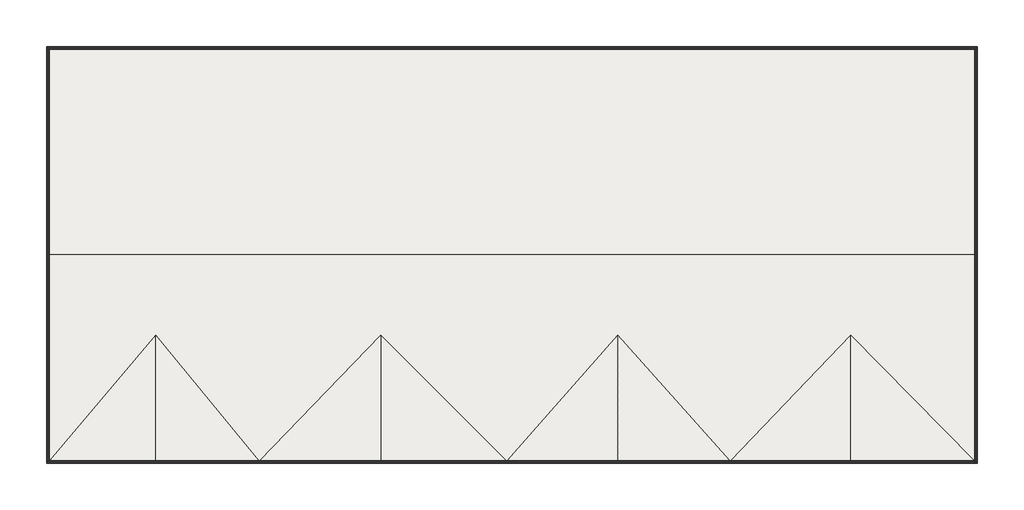
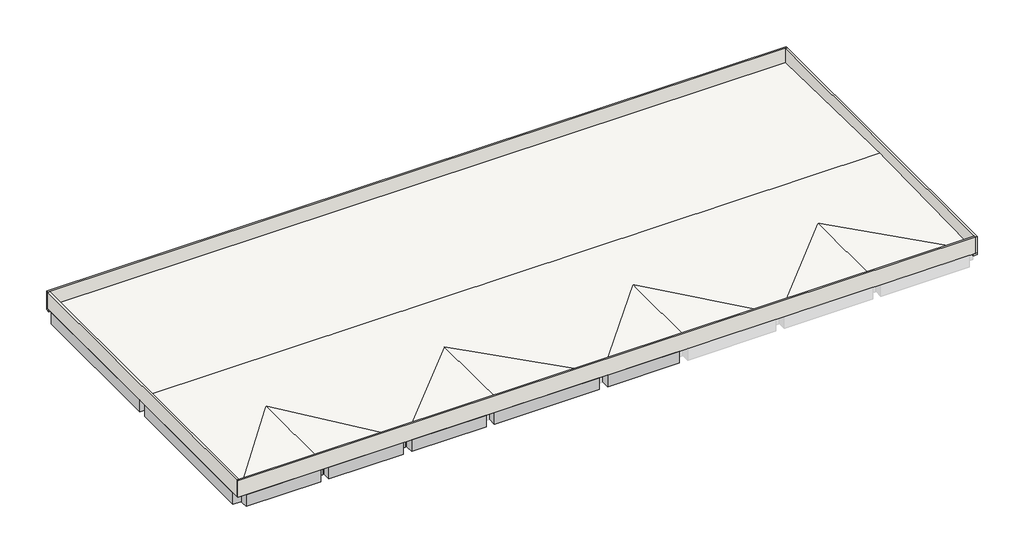
# One storey, part 1 of 2: 15 beams, 4 walls, 1 roof, 1 slab.
"""IFC4 building model written with IfcOpenShell, lengths in millimetres."""

from ifc_helpers import new_model, si_unit, frame, origin, place, context, project, spatial, polyline, outline, extrude, faceted_brep, element, save

model = new_model("IFC4")

# Units and contexts
model_context = context("Model", 3, world=origin())
ifc_project = project(units=[si_unit("LENGTHUNIT", "METRE", prefix="MILLI")], contexts=[model_context])

# Site, building, storey
site = spatial("IfcSite", under=ifc_project)
building = spatial("IfcBuilding", under=site)
storey = spatial("IfcBuildingStorey", under=building, Name="TOC", Elevation=104550.0)

# Beams
placement = place(None, origin())
element("IfcBeam", 1, ObjectType="RC Beam_Rectangular : H_SB_AR S16_RC Beam-AG_600x900_RG9", at=placement, inside=storey, context=model_context, shape_type="Brep", body=[
    faceted_brep([(300.0, -19200.0, 104550.0), (300.0, -19800.0, 104550.0), (5700.0, -19800.0, 104550.0), (5700.0, -19200.0, 104550.0), (3200.0, -19200.0, 104550.0), (2800.0, -19200.0, 104550.0), (300.0, -19800.0, 103650.0), (5700.0, -19800.0, 103650.0), (300.0, -19350.0, 103650.0), (300.0, -19200.0, 103650.0), (2800.0, -19200.0, 103650.0), (3200.0, -19200.0, 103650.0), (5700.0, -19200.0, 103650.0), (300.0, -19200.0, 104400.0)], [[[0, 1, 2, 3, 4, 5]], [[1, 6, 7, 2]], [[6, 8, 9, 10, 11, 12, 7]], [[9, 13, 0, 5, 4, 3, 12, 11, 10]], [[1, 0, 13, 9, 8, 6]], [[3, 2, 7, 12]]]),
])
element("IfcBeam", 2, ObjectType="RC Beam_Rectangular : H_SB_AR S16_RC Beam-AG_600x900_RG9", at=placement, inside=storey, context=model_context, shape_type="Brep", body=[
    faceted_brep([(6300.0, -19200.0, 104550.0), (6300.0, -19800.0, 104550.0), (11700.0, -19800.0, 104550.0), (11700.0, -19200.0, 104550.0), (9200.0, -19200.0, 104550.0), (8800.0, -19200.0, 104550.0), (6300.0, -19800.0, 103650.0), (11700.0, -19800.0, 103650.0), (6300.0, -19200.0, 103650.0), (8800.0, -19200.0, 103650.0), (9200.0, -19200.0, 103650.0), (11700.0, -19200.0, 103650.0)], [[[0, 1, 2, 3, 4, 5]], [[1, 6, 7, 2]], [[6, 8, 9, 10, 11, 7]], [[8, 0, 5, 4, 3, 11, 10, 9]], [[1, 0, 8, 6]], [[3, 2, 7, 11]]]),
])
element("IfcBeam", 3, ObjectType="RC Beam_Rectangular : H_SB_AR S16_RC Beam-AG_600x900_RG9", at=placement, inside=storey, context=model_context, shape_type="Brep", body=[
    faceted_brep([(12300.0, -19200.0, 104550.0), (12300.0, -19800.0, 104550.0), (17700.0, -19800.0, 104550.0), (17700.0, -19200.0, 104550.0), (15200.0, -19200.0, 104550.0), (14800.0, -19200.0, 104550.0), (12300.0, -19800.0, 103650.0), (17700.0, -19800.0, 103650.0), (12300.0, -19200.0, 103650.0), (14800.0, -19200.0, 103650.0), (15200.0, -19200.0, 103650.0), (17700.0, -19200.0, 103650.0), (17700.0, -19200.0, 104400.0)], [[[0, 1, 2, 3, 4, 5]], [[1, 6, 7, 2]], [[6, 8, 9, 10, 11, 7]], [[8, 0, 5, 4, 3, 12, 11, 10, 9]], [[1, 0, 8, 6]], [[3, 2, 7, 11, 12]]]),
])
element("IfcBeam", 4, ObjectType="RC Beam_Rectangular : H_SB_AR S16_RC Beam-AG_600x900_RG9", at=placement, inside=storey, context=model_context, shape_type="Brep", body=[
    faceted_brep([(18300.0, -19200.0, 104550.0), (18300.0, -19800.0, 104550.0), (25900.0, -19800.0, 104550.0), (25900.0, -19200.0, 104550.0), (22400.0, -19200.0, 104550.0), (21800.0, -19200.0, 104550.0), (25900.0, -19800.0, 103650.0), (18300.0, -19800.0, 103650.0), (18300.0, -19200.0, 103650.0), (21800.0, -19200.0, 103650.0), (22400.0, -19200.0, 103650.0), (25900.0, -19200.0, 103650.0), (18300.0, -19200.0, 104400.0)], [[[0, 1, 2, 3, 4, 5]], [[6, 2, 1, 7]], [[7, 8, 9, 10, 11, 6]], [[8, 12, 0, 5, 4, 3, 11, 10, 9]], [[0, 12, 8, 7, 1]], [[3, 2, 6, 11]]]),
])
element("IfcBeam", 5, ObjectType="RC Beam_Rectangular : H_SB_AR S16_RC Beam-AG_600x900_RG9", at=placement, inside=storey, context=model_context, shape_type="Brep", body=[
    faceted_brep([(26500.0, -19200.0, 104550.0), (26500.0, -19800.0, 104550.0), (31700.0, -19800.0, 104550.0), (31700.0, -19200.0, 104550.0), (29400.0, -19200.0, 104550.0), (28800.0, -19200.0, 104550.0), (26500.0, -19800.0, 103650.0), (31700.0, -19800.0, 103650.0), (26500.0, -19200.0, 103650.0), (28800.0, -19200.0, 103650.0), (29400.0, -19200.0, 103650.0), (31700.0, -19200.0, 103650.0)], [[[0, 1, 2, 3, 4, 5]], [[1, 6, 7, 2]], [[6, 8, 9, 10, 11, 7]], [[8, 0, 5, 4, 3, 11, 10, 9]], [[1, 0, 8, 6]], [[3, 2, 7, 11]]]),
])
element("IfcBeam", 6, ObjectType="RC Beam_Rectangular : H_SB_AR S16_RC Beam-AG_600x900_RG6", at=placement, inside=storey, context=model_context, shape_type="Brep", body=[
    faceted_brep([(-300.0, -19200.0, 104550.0), (300.0, -19200.0, 104550.0), (300.0, -8100.0, 104550.0), (-300.0, -8100.0, 104550.0), (300.0, -19200.0, 104400.0), (300.0, -19200.0, 103650.0), (300.0, -8100.0, 103650.0), (300.0, -8100.0, 104400.0), (150.0, -19200.0, 103650.0), (-300.0, -19200.0, 103650.0), (-300.0, -8100.0, 103650.0)], [[[0, 1, 2, 3]], [[1, 4, 5, 6, 7, 2]], [[5, 8, 9, 10, 6]], [[9, 0, 3, 10]], [[5, 4, 1, 0, 9, 8]], [[3, 2, 7, 6, 10]]]),
])
element("IfcBeam", 7, ObjectType="RC Beam_Rectangular : H_SB_AR S16_RC Beam-AG_600x900_RG6", at=placement, inside=storey, context=model_context, shape_type="Brep", body=[
    faceted_brep([(300.0, 3600.0, 104550.0), (-300.0, 3600.0, 104550.0), (-300.0, -7500.0, 104550.0), (300.0, -7500.0, 104550.0), (300.0, 3600.0, 103650.0), (300.0, 3600.0, 104400.0), (300.0, -7500.0, 104400.0), (300.0, -7500.0, 103650.0), (-300.0, 3600.0, 103650.0), (150.0, 3600.0, 103650.0), (-300.0, -7500.0, 103650.0)], [[[0, 1, 2, 3]], [[4, 5, 0, 3, 6, 7]], [[8, 9, 4, 7, 10]], [[10, 2, 1, 8]], [[0, 5, 4, 9, 8, 1]], [[3, 2, 10, 7, 6]]]),
])
element("IfcBeam", 8, ObjectType="RC Beam_Rectangular : H_SB_AR S16_RC Beam-AG_600x900_RG4", at=placement, inside=storey, context=model_context, shape_type="Brep", body=[
    faceted_brep([(300.0, -7500.0, 104550.0), (300.0, -8100.0, 104550.0), (2800.0, -8100.0, 104550.0), (3200.0, -8100.0, 104550.0), (5700.0, -8100.0, 104550.0), (5700.0, -7500.0, 104550.0), (3200.0, -7500.0, 104550.0), (2800.0, -7500.0, 104550.0), (300.0, -8100.0, 104400.0), (300.0, -8100.0, 103650.0), (2800.0, -8100.0, 103650.0), (3200.0, -8100.0, 103650.0), (5700.0, -8100.0, 103650.0), (300.0, -7900.0, 103650.0), (300.0, -7500.0, 103650.0), (2800.0, -7500.0, 103650.0), (3200.0, -7500.0, 103650.0), (5700.0, -7500.0, 103650.0), (300.0, -7500.0, 104400.0)], [[[0, 1, 2, 3, 4, 5, 6, 7]], [[1, 8, 9, 10, 11, 12, 4, 3, 2]], [[9, 13, 14, 15, 16, 17, 12, 11, 10]], [[14, 18, 0, 7, 6, 5, 17, 16, 15]], [[9, 8, 1, 0, 18, 14, 13]], [[5, 4, 12, 17]]]),
])
element("IfcBeam", 9, ObjectType="RC Beam_Rectangular : H_SB_AR S16_RC Beam-AG_400x900_RG1", at=placement, inside=storey, context=model_context, shape_type="Brep", body=[
    faceted_brep([(6200.0, -8100.0, 104550.0), (5800.0, -8100.0, 104550.0), (5800.0, -19200.0, 104550.0), (6200.0, -19200.0, 104550.0), (6200.0, -19200.0, 104400.0), (6200.0, -19200.0, 103650.0), (6200.0, -8100.0, 103650.0), (6200.0, -8100.0, 104400.0), (5800.0, -19200.0, 103650.0), (5800.0, -8100.0, 103650.0), (5800.0, -19200.0, 104400.0), (5800.0, -8100.0, 104400.0)], [[[0, 1, 2, 3]], [[3, 4, 5, 6, 7, 0]], [[8, 9, 6, 5]], [[8, 10, 2, 1, 11, 9]], [[2, 10, 8, 5, 4, 3]], [[0, 7, 6, 9, 11, 1]]]),
])
element("IfcBeam", 10, ObjectType="RC Beam_Rectangular : H_SB_AR S16_RC Beam-AG_400x900_RG1", at=placement, inside=storey, context=model_context, shape_type="Brep", body=[
    faceted_brep([(6200.0, 3600.0, 104550.0), (5800.0, 3600.0, 104550.0), (5800.0, -7500.0, 104550.0), (6200.0, -7500.0, 104550.0), (6200.0, -7500.0, 104400.0), (6200.0, -7500.0, 103650.0), (6200.0, 3600.0, 103650.0), (6200.0, 3600.0, 104400.0), (5800.0, -7500.0, 103650.0), (5800.0, 3600.0, 103650.0), (5800.0, -7500.0, 104400.0), (5800.0, 3600.0, 104400.0)], [[[0, 1, 2, 3]], [[3, 4, 5, 6, 7, 0]], [[8, 9, 6, 5]], [[8, 10, 2, 1, 11, 9]], [[2, 10, 8, 5, 4, 3]], [[0, 7, 6, 9, 11, 1]]]),
])
element("IfcBeam", 11, ObjectType="RC Beam_Rectangular : H_SB_AR S16_RC Beam-AG_400x900_RG1", at=placement, inside=storey, context=model_context, shape_type="Brep", body=[
    faceted_brep([(12200.0, -8100.0, 104550.0), (11800.0, -8100.0, 104550.0), (11800.0, -19200.0, 104550.0), (12200.0, -19200.0, 104550.0), (12200.0, -19200.0, 104400.0), (12200.0, -19200.0, 103650.0), (12200.0, -8100.0, 103650.0), (12200.0, -8100.0, 104400.0), (11800.0, -19200.0, 103650.0), (11800.0, -8100.0, 103650.0), (11800.0, -19200.0, 104400.0), (11800.0, -8100.0, 104400.0)], [[[0, 1, 2, 3]], [[3, 4, 5, 6, 7, 0]], [[8, 9, 6, 5]], [[8, 10, 2, 1, 11, 9]], [[2, 10, 8, 5, 4, 3]], [[0, 7, 6, 9, 11, 1]]]),
])
element("IfcBeam", 12, ObjectType="RC Beam_Rectangular : H_SB_AR S16_RC Beam-AG_400x900_RB1", at=placement, inside=storey, context=model_context, shape_type="Brep", body=[
    faceted_brep([(3200.0, 3600.0, 104550.0), (2800.0, 3600.0, 104550.0), (2800.0, -7500.0, 104550.0), (3200.0, -7500.0, 104550.0), (2800.0, 3600.0, 104400.0), (2800.0, 3600.0, 103650.0), (2800.0, -7500.0, 103650.0), (2800.0, -7500.0, 104400.0), (3200.0, 3600.0, 103650.0), (3200.0, -7500.0, 103650.0), (3200.0, 3600.0, 104400.0), (3200.0, -7500.0, 104400.0)], [[[0, 1, 2, 3]], [[1, 4, 5, 6, 7, 2]], [[5, 8, 9, 6]], [[8, 10, 0, 3, 11, 9]], [[1, 0, 10, 8, 5, 4]], [[3, 2, 7, 6, 9, 11]]]),
])
element("IfcBeam", 13, ObjectType="RC Beam_Rectangular : H_SB_AR S16_RC Beam-AG_400x900_RB1", at=placement, inside=storey, context=model_context, shape_type="Brep", body=[
    faceted_brep([(2800.0, -19200.0, 104550.0), (3200.0, -19200.0, 104550.0), (3200.0, -8100.0, 104550.0), (2800.0, -8100.0, 104550.0), (2800.0, -19200.0, 103650.0), (2800.0, -19200.0, 104400.0), (2800.0, -8100.0, 104400.0), (2800.0, -8100.0, 103650.0), (3200.0, -19200.0, 103650.0), (3200.0, -8100.0, 103650.0), (3200.0, -19200.0, 104400.0), (3200.0, -8100.0, 104400.0)], [[[0, 1, 2, 3]], [[4, 5, 0, 3, 6, 7]], [[8, 4, 7, 9]], [[1, 10, 8, 9, 11, 2]], [[1, 0, 5, 4, 8, 10]], [[3, 2, 11, 9, 7, 6]]]),
])
element("IfcBeam", 14, ObjectType="RC Beam_Rectangular : H_SB_AR S16_RC Beam-AG_400x900_RB1", at=placement, inside=storey, context=model_context, shape_type="Brep", body=[
    faceted_brep([(8800.0, -19200.0, 104550.0), (9200.0, -19200.0, 104550.0), (9200.0, -8100.0, 104550.0), (8800.0, -8100.0, 104550.0), (8800.0, -19200.0, 103650.0), (8800.0, -19200.0, 104400.0), (8800.0, -8100.0, 104400.0), (8800.0, -8100.0, 103650.0), (9200.0, -19200.0, 103650.0), (9200.0, -8100.0, 103650.0), (9200.0, -19200.0, 104400.0), (9200.0, -8100.0, 104400.0)], [[[0, 1, 2, 3]], [[4, 5, 0, 3, 6, 7]], [[8, 4, 7, 9]], [[1, 10, 8, 9, 11, 2]], [[1, 0, 5, 4, 8, 10]], [[3, 2, 11, 9, 7, 6]]]),
])
element("IfcBeam", 15, ObjectType="RC Beam_Rectangular : H_SB_AR S16_RC Beam-AG_400x900_RB1", at=placement, inside=storey, context=model_context, shape_type="Brep", body=[
    faceted_brep([(14800.0, -19200.0, 104550.0), (15200.0, -19200.0, 104550.0), (15200.0, -8100.0, 104550.0), (14800.0, -8100.0, 104550.0), (14800.0, -19200.0, 103650.0), (14800.0, -19200.0, 104400.0), (14800.0, -8100.0, 104400.0), (14800.0, -8100.0, 103650.0), (15200.0, -19200.0, 103650.0), (15200.0, -8100.0, 103650.0), (15200.0, -19200.0, 104400.0), (15200.0, -8100.0, 104400.0)], [[[0, 1, 2, 3]], [[4, 5, 0, 3, 6, 7]], [[8, 4, 7, 9]], [[1, 10, 8, 9, 11, 2]], [[1, 0, 5, 4, 8, 10]], [[3, 2, 11, 9, 7, 6]]]),
])

# Roof
element("IfcRoof", 16, ObjectType="H_RF_AR B06_RC Roof Finish_Type1", at=placement, inside=storey, context=model_context, shape_type="Brep", body=[
    faceted_brep([(53150.0, -19650.0, 104550.0), (-150.0, -19650.0, 104550.0), (-150.0, 4050.0, 104550.0), (53150.0, 4050.0, 104550.0), (-150.0, -19650.0, 104720.0), (53150.0, -19650.0, 104720.0), (46000.0, -19650.0, 104866.0), (39071.6723549, -19650.0, 104720.0), (32600.0, -19650.0, 104866.0), (26200.0, -19650.0, 104720.0), (18950.0, -19650.0, 104866.0), (11938.5665529, -19650.0, 104720.0), (6000.0, -19650.0, 104866.0), (-150.0, 4050.0, 104720.0), (-150.0, -7800.0, 104959.0), (53150.0, 4050.0, 104720.0), (53150.0, -7800.0, 104959.0), (6000.0, -12400.0, 104866.2236287), (18950.0, -12400.0, 104866.2236287), (32600.0, -12400.0, 104866.2236287), (46000.0, -12400.0, 104866.2236287)], [[[0, 1, 2, 3]], [[4, 1, 0, 5, 6, 7, 8, 9, 10, 11, 12]], [[13, 2, 1, 4, 14]], [[15, 3, 2, 13]], [[5, 0, 3, 15, 16]], [[5, 16, 14, 4, 17, 11, 18, 9, 19, 7, 20]], [[15, 13, 14, 16]], [[5, 20, 6]], [[20, 7, 6]], [[4, 12, 17]], [[17, 12, 11]], [[11, 10, 18]], [[18, 10, 9]], [[9, 8, 19]], [[7, 19, 8]]]),
])

# Slab
element("IfcSlab", 17, ObjectType="H_FL_AR_S17_RC Slab_RS1 T150", at=placement, inside=storey, context=model_context, shape_type="Brep", body=[
    faceted_brep([(-300.0, 4200.0, 104400.0), (0.0, 4200.0, 104400.0), (0.0, 3900.0, 104400.0), (-300.0, 3900.0, 104400.0), (0.0, 4200.0, 104550.0), (-300.0, 4200.0, 104550.0), (-300.0, 3900.0, 104550.0), (0.0, 3900.0, 104550.0)], [[[0, 1, 2, 3]], [[4, 5, 6, 7]], [[5, 0, 3, 6]], [[0, 5, 4, 1]], [[1, 4, 7, 2]], [[3, 2, 7, 6]]]),
    faceted_brep([(53300.0, -19800.0, 104400.0), (53000.0, -19800.0, 104400.0), (53000.0, -19500.0, 104400.0), (53300.0, -19500.0, 104400.0), (53000.0, -19800.0, 104550.0), (53300.0, -19800.0, 104550.0), (53300.0, -19500.0, 104550.0), (53000.0, -19500.0, 104550.0)], [[[0, 1, 2, 3]], [[4, 5, 6, 7]], [[0, 5, 4, 1]], [[5, 0, 3, 6]], [[1, 4, 7, 2]], [[3, 2, 7, 6]]]),
    faceted_brep([(53300.0, 4200.0, 104400.0), (53300.0, 3900.0, 104400.0), (53000.0, 3900.0, 104400.0), (53000.0, 4200.0, 104400.0), (53300.0, 3900.0, 104550.0), (53300.0, 4200.0, 104550.0), (53000.0, 4200.0, 104550.0), (53000.0, 3900.0, 104550.0)], [[[0, 1, 2, 3]], [[4, 5, 6, 7]], [[5, 0, 3, 6]], [[0, 5, 4, 1]], [[6, 3, 2, 7]], [[2, 1, 4, 7]]]),
    faceted_brep([(17700.0, -8100.0, 104400.0), (17700.0, -19200.0, 104400.0), (15200.0, -19200.0, 104400.0), (15200.0, -8100.0, 104400.0), (15200.0, -19200.0, 104550.0), (17700.0, -19200.0, 104550.0), (17700.0, -8100.0, 104550.0), (15200.0, -8100.0, 104550.0)], [[[0, 1, 2, 3]], [[4, 5, 6, 7]], [[1, 5, 4, 2]], [[5, 1, 0, 6]], [[6, 0, 3, 7]], [[3, 2, 4, 7]]]),
    faceted_brep([(17700.0, 3600.0, 104400.0), (17700.0, -7500.0, 104400.0), (15200.0, -7500.0, 104400.0), (15200.0, 3600.0, 104400.0), (17700.0, -7500.0, 104550.0), (17700.0, 3600.0, 104550.0), (15200.0, 3600.0, 104550.0), (15200.0, -7500.0, 104550.0)], [[[0, 1, 2, 3]], [[4, 5, 6, 7]], [[5, 0, 3, 6]], [[1, 4, 7, 2]], [[1, 0, 5, 4]], [[3, 2, 7, 6]]]),
    faceted_brep([(6200.0, -19200.0, 104400.0), (6200.0, -8100.0, 104400.0), (8800.0, -8100.0, 104400.0), (8800.0, -19200.0, 104400.0), (6200.0, -8100.0, 104550.0), (6200.0, -19200.0, 104550.0), (6300.0, -19200.0, 104550.0), (8800.0, -19200.0, 104550.0), (8800.0, -8100.0, 104550.0), (6300.0, -8100.0, 104550.0)], [[[0, 1, 2, 3]], [[4, 5, 6, 7, 8, 9]], [[5, 0, 3, 7, 6]], [[1, 4, 9, 8, 2]], [[1, 0, 5, 4]], [[3, 2, 8, 7]]]),
    faceted_brep([(5800.0, -8100.0, 104400.0), (5800.0, -19200.0, 104400.0), (3200.0, -19200.0, 104400.0), (3200.0, -8100.0, 104400.0), (5800.0, -19200.0, 104550.0), (5800.0, -8100.0, 104550.0), (5700.0, -8100.0, 104550.0), (3200.0, -8100.0, 104550.0), (3200.0, -19200.0, 104550.0), (5700.0, -19200.0, 104550.0)], [[[0, 1, 2, 3]], [[4, 5, 6, 7, 8, 9]], [[1, 4, 9, 8, 2]], [[5, 0, 3, 7, 6]], [[1, 0, 5, 4]], [[3, 2, 8, 7]]]),
    faceted_brep([(6200.0, -7500.0, 104400.0), (6200.0, 3600.0, 104400.0), (8800.0, 3600.0, 104400.0), (8800.0, -7500.0, 104400.0), (6200.0, 3600.0, 104550.0), (6200.0, -7500.0, 104550.0), (6300.0, -7500.0, 104550.0), (8800.0, -7500.0, 104550.0), (8800.0, 3600.0, 104550.0), (6300.0, 3600.0, 104550.0)], [[[0, 1, 2, 3]], [[4, 5, 6, 7, 8, 9]], [[1, 4, 9, 8, 2]], [[5, 0, 3, 7, 6]], [[1, 0, 5, 4]], [[3, 2, 8, 7]]]),
    faceted_brep([(5800.0, 3600.0, 104400.0), (5800.0, -7500.0, 104400.0), (3200.0, -7500.0, 104400.0), (3200.0, 3600.0, 104400.0), (5800.0, -7500.0, 104550.0), (5800.0, 3600.0, 104550.0), (5700.0, 3600.0, 104550.0), (3200.0, 3600.0, 104550.0), (3200.0, -7500.0, 104550.0), (5700.0, -7500.0, 104550.0)], [[[0, 1, 2, 3]], [[4, 5, 6, 7, 8, 9]], [[5, 0, 3, 7, 6]], [[1, 4, 9, 8, 2]], [[1, 0, 5, 4]], [[3, 2, 8, 7]]]),
    faceted_brep([(12200.0, -19200.0, 104400.0), (12200.0, -8100.0, 104400.0), (14800.0, -8100.0, 104400.0), (14800.0, -19200.0, 104400.0), (12200.0, -8100.0, 104550.0), (12200.0, -19200.0, 104550.0), (12300.0, -19200.0, 104550.0), (14800.0, -19200.0, 104550.0), (14800.0, -8100.0, 104550.0), (12300.0, -8100.0, 104550.0)], [[[0, 1, 2, 3]], [[4, 5, 6, 7, 8, 9]], [[5, 0, 3, 7, 6]], [[1, 4, 9, 8, 2]], [[1, 0, 5, 4]], [[3, 2, 8, 7]]]),
    faceted_brep([(11800.0, -8100.0, 104400.0), (11800.0, -19200.0, 104400.0), (9200.0, -19200.0, 104400.0), (9200.0, -8100.0, 104400.0), (11800.0, -19200.0, 104550.0), (11800.0, -8100.0, 104550.0), (11700.0, -8100.0, 104550.0), (9200.0, -8100.0, 104550.0), (9200.0, -19200.0, 104550.0), (11700.0, -19200.0, 104550.0)], [[[0, 1, 2, 3]], [[4, 5, 6, 7, 8, 9]], [[1, 4, 9, 8, 2]], [[5, 0, 3, 7, 6]], [[1, 0, 5, 4]], [[3, 2, 8, 7]]]),
    faceted_brep([(12200.0, -7500.0, 104400.0), (12200.0, 3600.0, 104400.0), (14800.0, 3600.0, 104400.0), (14800.0, -7500.0, 104400.0), (12200.0, 3600.0, 104550.0), (12200.0, -7500.0, 104550.0), (12300.0, -7500.0, 104550.0), (14800.0, -7500.0, 104550.0), (14800.0, 3600.0, 104550.0), (12300.0, 3600.0, 104550.0)], [[[0, 1, 2, 3]], [[4, 5, 6, 7, 8, 9]], [[1, 4, 9, 8, 2]], [[5, 0, 3, 7, 6]], [[1, 0, 5, 4]], [[3, 2, 8, 7]]]),
    faceted_brep([(11800.0, 3600.0, 104400.0), (11800.0, -7500.0, 104400.0), (9200.0, -7500.0, 104400.0), (9200.0, 3600.0, 104400.0), (11800.0, -7500.0, 104550.0), (11800.0, 3600.0, 104550.0), (11700.0, 3600.0, 104550.0), (9200.0, 3600.0, 104550.0), (9200.0, -7500.0, 104550.0), (11700.0, -7500.0, 104550.0)], [[[0, 1, 2, 3]], [[4, 5, 6, 7, 8, 9]], [[5, 0, 3, 7, 6]], [[1, 4, 9, 8, 2]], [[1, 0, 5, 4]], [[3, 2, 8, 7]]]),
    faceted_brep([(2800.0, -8100.0, 104400.0), (2800.0, -19200.0, 104400.0), (426.0, -19200.0, 104400.0), (300.0, -19200.0, 104400.0), (300.0, -8100.0, 104400.0), (426.0, -8100.0, 104400.0), (300.0, -19200.0, 104550.0), (2800.0, -19200.0, 104550.0), (2800.0, -8100.0, 104550.0), (300.0, -8100.0, 104550.0)], [[[0, 1, 2, 3, 4, 5]], [[6, 7, 8, 9]], [[6, 3, 2, 1, 7]], [[3, 6, 9, 4]], [[4, 9, 8, 0, 5]], [[1, 0, 8, 7]]]),
    faceted_brep([(25950.0, 3600.0, 104400.0), (25950.0, -11400.0, 104400.0), (22400.0, -11400.0, 104400.0), (22400.0, 3600.0, 104400.0), (25950.0, -11400.0, 104550.0), (25950.0, 3600.0, 104550.0), (25900.0, 3600.0, 104550.0), (22400.0, 3600.0, 104550.0), (22400.0, -11400.0, 104550.0), (25900.0, -11400.0, 104550.0)], [[[0, 1, 2, 3]], [[4, 5, 6, 7, 8, 9]], [[5, 0, 3, 7, 6]], [[1, 4, 9, 8, 2]], [[1, 0, 5, 4]], [[3, 2, 8, 7]]]),
    faceted_brep([(26450.0, -11400.0, 104400.0), (26450.0, 3600.0, 104400.0), (28800.0, 3600.0, 104400.0), (28800.0, -11400.0, 104400.0), (26450.0, 3600.0, 104550.0), (26450.0, -11400.0, 104550.0), (26500.0, -11400.0, 104550.0), (28800.0, -11400.0, 104550.0), (28800.0, 3600.0, 104550.0), (26500.0, 3600.0, 104550.0)], [[[0, 1, 2, 3]], [[4, 5, 6, 7, 8, 9]], [[1, 4, 9, 8, 2]], [[5, 0, 3, 7, 6]], [[1, 0, 5, 4]], [[3, 2, 8, 7]]]),
    faceted_brep([(25950.0, -12000.0, 104400.0), (25950.0, -19200.0, 104400.0), (22400.0, -19200.0, 104400.0), (22400.0, -12000.0, 104400.0), (25950.0, -19200.0, 104550.0), (25950.0, -12000.0, 104550.0), (25900.0, -12000.0, 104550.0), (22400.0, -12000.0, 104550.0), (22400.0, -19200.0, 104550.0), (25900.0, -19200.0, 104550.0)], [[[0, 1, 2, 3]], [[4, 5, 6, 7, 8, 9]], [[1, 4, 9, 8, 2]], [[5, 0, 3, 7, 6]], [[1, 0, 5, 4]], [[3, 2, 8, 7]]]),
    faceted_brep([(31750.0, 3600.0, 104400.0), (31750.0, -11400.0, 104400.0), (29400.0, -11400.0, 104400.0), (29400.0, 3600.0, 104400.0), (31750.0, -11400.0, 104550.0), (31750.0, 3600.0, 104550.0), (31700.0, 3600.0, 104550.0), (29400.0, 3600.0, 104550.0), (29400.0, -11400.0, 104550.0), (31700.0, -11400.0, 104550.0)], [[[0, 1, 2, 3]], [[4, 5, 6, 7, 8, 9]], [[5, 0, 3, 7, 6]], [[1, 4, 9, 8, 2]], [[1, 0, 5, 4]], [[3, 2, 8, 7]]]),
    faceted_brep([(32250.0, -11400.0, 104400.0), (32250.0, 3600.0, 104400.0), (33250.0, 3600.0, 104400.0), (33450.0, 3600.0, 104400.0), (35200.0, 3600.0, 104400.0), (35200.0, -11400.0, 104400.0), (33450.0, -11400.0, 104400.0), (33250.0, -11400.0, 104400.0), (32250.0, 3600.0, 104550.0), (32250.0, -11400.0, 104550.0), (32300.0, -11400.0, 104550.0), (35200.0, -11400.0, 104550.0), (35200.0, 3600.0, 104550.0), (32300.0, 3600.0, 104550.0)], [[[0, 1, 2, 3, 4, 5, 6, 7]], [[8, 9, 10, 11, 12, 13]], [[1, 8, 13, 12, 4, 3, 2]], [[9, 0, 7, 6, 5, 11, 10]], [[1, 0, 9, 8]], [[5, 4, 12, 11]]]),
    faceted_brep([(32250.0, -19200.0, 104400.0), (32250.0, -12000.0, 104400.0), (35200.0, -12000.0, 104400.0), (35200.0, -19200.0, 104400.0), (32250.0, -12000.0, 104550.0), (32250.0, -19200.0, 104550.0), (32300.0, -19200.0, 104550.0), (35200.0, -19200.0, 104550.0), (35200.0, -12000.0, 104550.0), (32300.0, -12000.0, 104550.0)], [[[0, 1, 2, 3]], [[4, 5, 6, 7, 8, 9]], [[5, 0, 3, 7, 6]], [[1, 4, 9, 8, 2]], [[1, 0, 5, 4]], [[3, 2, 8, 7]]]),
    faceted_brep([(26450.0, -19200.0, 104400.0), (26450.0, -12000.0, 104400.0), (26500.0, -12000.0, 104400.0), (28500.0, -12000.0, 104400.0), (28700.0, -12000.0, 104400.0), (28800.0, -12000.0, 104400.0), (28800.0, -15000.0, 104400.0), (28800.0, -15200.0, 104400.0), (28800.0, -19200.0, 104400.0), (28700.0, -19200.0, 104400.0), (28500.0, -19200.0, 104400.0), (26500.0, -19200.0, 104400.0), (26450.0, -12000.0, 104550.0), (26450.0, -19200.0, 104550.0), (26500.0, -19200.0, 104550.0), (28800.0, -19200.0, 104550.0), (28800.0, -12000.0, 104550.0), (26500.0, -12000.0, 104550.0)], [[[0, 1, 2, 3, 4, 5, 6, 7, 8, 9, 10, 11]], [[12, 13, 14, 15, 16, 17]], [[13, 0, 11, 10, 9, 8, 15, 14]], [[1, 12, 17, 16, 5, 4, 3, 2]], [[1, 0, 13, 12]], [[8, 7, 6, 5, 16, 15]]]),
    faceted_brep([(31750.0, -12000.0, 104400.0), (31750.0, -19200.0, 104400.0), (31700.0, -19200.0, 104400.0), (29400.0, -19200.0, 104400.0), (29400.0, -15200.0, 104400.0), (29400.0, -15000.0, 104400.0), (29400.0, -12000.0, 104400.0), (31700.0, -12000.0, 104400.0), (31750.0, -19200.0, 104550.0), (31750.0, -12000.0, 104550.0), (31700.0, -12000.0, 104550.0), (29400.0, -12000.0, 104550.0), (29400.0, -19200.0, 104550.0), (31700.0, -19200.0, 104550.0)], [[[0, 1, 2, 3, 4, 5, 6, 7]], [[8, 9, 10, 11, 12, 13]], [[1, 8, 13, 12, 3, 2]], [[9, 0, 7, 6, 11, 10]], [[1, 0, 9, 8]], [[6, 5, 4, 3, 12, 11]]]),
    faceted_brep([(38750.0, 3600.0, 104400.0), (38750.0, -9150.0, 104400.0), (38750.0, -9350.0, 104400.0), (38750.0, -11400.0, 104400.0), (36700.0, -11400.0, 104400.0), (36500.0, -11400.0, 104400.0), (35800.0, -11400.0, 104400.0), (35800.0, 3600.0, 104400.0), (38750.0, -11400.0, 104550.0), (38750.0, 3600.0, 104550.0), (38700.0, 3600.0, 104550.0), (35800.0, 3600.0, 104550.0), (35800.0, -11400.0, 104550.0), (38700.0, -11400.0, 104550.0)], [[[0, 1, 2, 3, 4, 5, 6, 7]], [[8, 9, 10, 11, 12, 13]], [[9, 0, 7, 11, 10]], [[3, 8, 13, 12, 6, 5, 4]], [[3, 2, 1, 0, 9, 8]], [[7, 6, 12, 11]]]),
    faceted_brep([(39250.0, -11400.0, 104400.0), (39250.0, -9350.0, 104400.0), (39250.0, -9150.0, 104400.0), (39250.0, 3600.0, 104400.0), (42200.0, 3600.0, 104400.0), (42200.0, -9150.0, 104400.0), (42200.0, -9350.0, 104400.0), (42200.0, -11400.0, 104400.0), (39250.0, 3600.0, 104550.0), (39250.0, -11400.0, 104550.0), (39300.0, -11400.0, 104550.0), (42200.0, -11400.0, 104550.0), (42200.0, 3600.0, 104550.0), (39300.0, 3600.0, 104550.0)], [[[0, 1, 2, 3, 4, 5, 6, 7]], [[8, 9, 10, 11, 12, 13]], [[3, 8, 13, 12, 4]], [[9, 0, 7, 11, 10]], [[3, 2, 1, 0, 9, 8]], [[7, 6, 5, 4, 12, 11]]]),
    faceted_brep([(38750.0, -12000.0, 104400.0), (38750.0, -19200.0, 104400.0), (38700.0, -19200.0, 104400.0), (36700.0, -19200.0, 104400.0), (36500.0, -19200.0, 104400.0), (35800.0, -19200.0, 104400.0), (35800.0, -12000.0, 104400.0), (36500.0, -12000.0, 104400.0), (36700.0, -12000.0, 104400.0), (38700.0, -12000.0, 104400.0), (38750.0, -19200.0, 104550.0), (38750.0, -12000.0, 104550.0), (38700.0, -12000.0, 104550.0), (35800.0, -12000.0, 104550.0), (35800.0, -19200.0, 104550.0), (38700.0, -19200.0, 104550.0)], [[[0, 1, 2, 3, 4, 5, 6, 7, 8, 9]], [[10, 11, 12, 13, 14, 15]], [[1, 10, 15, 14, 5, 4, 3, 2]], [[11, 0, 9, 8, 7, 6, 13, 12]], [[1, 0, 11, 10]], [[6, 5, 14, 13]]]),
    faceted_brep([(39250.0, -19200.0, 104400.0), (39250.0, -15350.0, 104400.0), (39250.0, -15150.0, 104400.0), (39250.0, -12000.0, 104400.0), (42100.0, -12000.0, 104400.0), (42200.0, -12000.0, 104400.0), (42200.0, -15150.0, 104400.0), (42200.0, -15350.0, 104400.0), (42200.0, -19200.0, 104400.0), (39250.0, -12000.0, 104550.0), (39250.0, -19200.0, 104550.0), (39300.0, -19200.0, 104550.0), (42200.0, -19200.0, 104550.0), (42200.0, -12000.0, 104550.0), (39300.0, -12000.0, 104550.0)], [[[0, 1, 2, 3, 4, 5, 6, 7, 8]], [[9, 10, 11, 12, 13, 14]], [[10, 0, 8, 12, 11]], [[3, 9, 14, 13, 5, 4]], [[3, 2, 1, 0, 10, 9]], [[8, 7, 6, 5, 13, 12]]]),
    faceted_brep([(45750.0, 3600.0, 104400.0), (45750.0, 900.0, 104400.0), (45750.0, 700.0, 104400.0), (45750.0, -9150.0, 104400.0), (45750.0, -9350.0, 104400.0), (45750.0, -11400.0, 104400.0), (42800.0, -11400.0, 104400.0), (42800.0, -9350.0, 104400.0), (42800.0, -9150.0, 104400.0), (42800.0, 3600.0, 104400.0), (43550.0, 3600.0, 104400.0), (43600.0, 3600.0, 104400.0), (43800.0, 3600.0, 104400.0), (45750.0, -11400.0, 104550.0), (45750.0, 3600.0, 104550.0), (45700.0, 3600.0, 104550.0), (42800.0, 3600.0, 104550.0), (42800.0, -11400.0, 104550.0), (45700.0, -11400.0, 104550.0)], [[[0, 1, 2, 3, 4, 5, 6, 7, 8, 9, 10, 11, 12]], [[13, 14, 15, 16, 17, 18]], [[14, 0, 12, 11, 10, 9, 16, 15]], [[5, 13, 18, 17, 6]], [[5, 4, 3, 2, 1, 0, 14, 13]], [[9, 8, 7, 6, 17, 16]]]),
    faceted_brep([(46250.0, -11400.0, 104400.0), (46250.0, -10150.0, 104400.0), (46250.0, -9950.0, 104400.0), (46250.0, -6215.0, 104400.0), (46250.0, -6015.0, 104400.0), (46250.0, -4945.0, 104400.0), (46250.0, -4745.0, 104400.0), (46250.0, -3565.0, 104400.0), (46250.0, -3365.0, 104400.0), (46250.0, -1950.0, 104400.0), (46250.0, -1750.0, 104400.0), (46250.0, -550.0, 104400.0), (46250.0, -350.0, 104400.0), (46250.0, 3600.0, 104400.0), (46600.0, 3600.0, 104400.0), (46600.0, -1750.0, 104400.0), (46600.0, -1950.0, 104400.0), (46600.0, -6015.0, 104400.0), (46600.0, -6215.0, 104400.0), (46600.0, -9950.0, 104400.0), (46600.0, -10150.0, 104400.0), (46600.0, -11400.0, 104400.0), (46250.0, 3600.0, 104550.0), (46250.0, -11400.0, 104550.0), (46300.0, -11400.0, 104550.0), (46600.0, -11400.0, 104550.0), (46600.0, 3600.0, 104550.0), (46300.0, 3600.0, 104550.0)], [[[0, 1, 2, 3, 4, 5, 6, 7, 8, 9, 10, 11, 12, 13, 14, 15, 16, 17, 18, 19, 20, 21]], [[22, 23, 24, 25, 26, 27]], [[13, 22, 27, 26, 14]], [[23, 0, 21, 25, 24]], [[13, 12, 11, 10, 9, 8, 7, 6, 5, 4, 3, 2, 1, 0, 23, 22]], [[21, 20, 19, 18, 17, 16, 15, 14, 26, 25]]]),
    faceted_brep([(45750.0, -12000.0, 104400.0), (45750.0, -13200.0, 104400.0), (45750.0, -13400.0, 104400.0), (45750.0, -15150.0, 104400.0), (45750.0, -15350.0, 104400.0), (45750.0, -19200.0, 104400.0), (43500.0, -19200.0, 104400.0), (43300.0, -19200.0, 104400.0), (43100.0, -19200.0, 104400.0), (42800.0, -19200.0, 104400.0), (42800.0, -15350.0, 104400.0), (42800.0, -15150.0, 104400.0), (42800.0, -13899.2374861, 104400.0), (42800.0, -13699.2374861, 104400.0), (42800.0, -12000.0, 104400.0), (43300.0, -12000.0, 104400.0), (43500.0, -12000.0, 104400.0), (45000.0, -12000.0, 104400.0), (45200.0, -12000.0, 104400.0), (45750.0, -19200.0, 104550.0), (45750.0, -12000.0, 104550.0), (45700.0, -12000.0, 104550.0), (42800.0, -12000.0, 104550.0), (42800.0, -19200.0, 104550.0), (45700.0, -19200.0, 104550.0)], [[[0, 1, 2, 3, 4, 5, 6, 7, 8, 9, 10, 11, 12, 13, 14, 15, 16, 17, 18]], [[19, 20, 21, 22, 23, 24]], [[5, 19, 24, 23, 9, 8, 7, 6]], [[20, 0, 18, 17, 16, 15, 14, 22, 21]], [[5, 4, 3, 2, 1, 0, 20, 19]], [[14, 13, 12, 11, 10, 9, 23, 22]]]),
    faceted_brep([(46250.0, -19200.0, 104400.0), (46250.0, -15350.0, 104400.0), (46250.0, -15150.0, 104400.0), (46250.0, -13400.0, 104400.0), (46250.0, -13200.0, 104400.0), (46250.0, -12000.0, 104400.0), (46600.0, -12000.0, 104400.0), (47200.0, -12000.0, 104400.0), (49200.0, -12000.0, 104400.0), (49200.0, -19200.0, 104400.0), (46800.0, -19200.0, 104400.0), (46600.0, -19200.0, 104400.0), (46250.0, -12000.0, 104550.0), (46250.0, -19200.0, 104550.0), (46300.0, -19200.0, 104550.0), (49200.0, -19200.0, 104550.0), (49200.0, -12000.0, 104550.0), (47200.0, -12000.0, 104550.0), (46600.0, -12000.0, 104550.0), (46300.0, -12000.0, 104550.0)], [[[0, 1, 2, 3, 4, 5, 6, 7, 8, 9, 10, 11]], [[12, 13, 14, 15, 16, 17, 18, 19]], [[13, 0, 11, 10, 9, 15, 14]], [[5, 12, 19, 18, 17, 16, 8, 7, 6]], [[5, 4, 3, 2, 1, 0, 13, 12]], [[9, 8, 16, 15]]]),
    faceted_brep([(300.0, 3600.0, 104400.0), (426.0, 3600.0, 104400.0), (2800.0, 3600.0, 104400.0), (2800.0, -7500.0, 104400.0), (300.0, -7500.0, 104400.0), (2800.0, -7500.0, 104550.0), (2800.0, 3600.0, 104550.0), (300.0, 3600.0, 104550.0), (300.0, -7500.0, 104550.0)], [[[0, 1, 2, 3, 4]], [[5, 6, 7, 8]], [[0, 7, 6, 2, 1]], [[7, 0, 4, 8]], [[8, 4, 3, 5]], [[3, 2, 6, 5]]]),
    faceted_brep([(18300.0, -11400.0, 104400.0), (18300.0, 3474.0, 104400.0), (18300.0, 3600.0, 104400.0), (21800.0, 3600.0, 104400.0), (21800.0, -11400.0, 104400.0), (21800.0, -11400.0, 104550.0), (21800.0, 3600.0, 104550.0), (18300.0, 3600.0, 104550.0), (18300.0, -7500.0, 104550.0), (18300.0, -8100.0, 104550.0), (18300.0, -11400.0, 104550.0)], [[[0, 1, 2, 3, 4]], [[5, 6, 7, 8, 9, 10]], [[2, 7, 6, 3]], [[10, 0, 4, 5]], [[0, 10, 9, 8, 7, 2, 1]], [[4, 3, 6, 5]]]),
    faceted_brep([(52700.0, 3600.0, 104400.0), (52700.0, 3474.0, 104400.0), (52700.0, -1750.0, 104400.0), (52700.0, -1950.0, 104400.0), (52700.0, -6015.0, 104400.0), (52700.0, -6215.0, 104400.0), (52700.0, -8200.0, 104400.0), (52700.0, -8400.0, 104400.0), (52700.0, -11400.0, 104400.0), (52574.0, -11400.0, 104400.0), (52374.0, -11400.0, 104400.0), (50570.0, -11400.0, 104400.0), (50370.0, -11400.0, 104400.0), (49800.0, -11400.0, 104400.0), (49200.0, -11400.0, 104400.0), (47200.0, -11400.0, 104400.0), (47200.0, -10150.0, 104400.0), (47200.0, -9950.0, 104400.0), (47200.0, -6215.0, 104400.0), (47200.0, -6015.0, 104400.0), (47200.0, -1950.0, 104400.0), (47200.0, -1750.0, 104400.0), (47200.0, 3600.0, 104400.0), (48900.0, 3600.0, 104400.0), (49100.0, 3600.0, 104400.0), (47200.0, 3600.0, 104550.0), (47200.0, -11400.0, 104550.0), (49200.0, -11400.0, 104550.0), (49800.0, -11400.0, 104550.0), (52700.0, -11400.0, 104550.0), (52700.0, 3600.0, 104550.0)], [[[0, 1, 2, 3, 4, 5, 6, 7, 8, 9, 10, 11, 12, 13, 14, 15, 16, 17, 18, 19, 20, 21, 22, 23, 24]], [[25, 26, 27, 28, 29, 30]], [[30, 0, 24, 23, 22, 25]], [[0, 30, 29, 8, 7, 6, 5, 4, 3, 2, 1]], [[8, 29, 28, 27, 26, 15, 14, 13, 12, 11, 10, 9]], [[22, 21, 20, 19, 18, 17, 16, 15, 26, 25]]]),
    faceted_brep([(52700.0, -12000.0, 104400.0), (52700.0, -19200.0, 104400.0), (52574.0, -19200.0, 104400.0), (49800.0, -19200.0, 104400.0), (49800.0, -12000.0, 104400.0), (49800.0, -19200.0, 104550.0), (52700.0, -19200.0, 104550.0), (52700.0, -12000.0, 104550.0), (49800.0, -12000.0, 104550.0)], [[[0, 1, 2, 3, 4]], [[5, 6, 7, 8]], [[1, 6, 5, 3, 2]], [[6, 1, 0, 7]], [[7, 0, 4, 8]], [[4, 3, 5, 8]]]),
    faceted_brep([(18300.0, -19200.0, 104400.0), (18300.0, -19074.0, 104400.0), (18300.0, -12000.0, 104400.0), (21800.0, -12000.0, 104400.0), (21800.0, -19200.0, 104400.0), (18300.0, -12000.0, 104550.0), (18300.0, -19200.0, 104550.0), (21800.0, -19200.0, 104550.0), (21800.0, -12000.0, 104550.0)], [[[0, 1, 2, 3, 4]], [[5, 6, 7, 8]], [[6, 0, 4, 7]], [[2, 5, 8, 3]], [[2, 1, 0, 6, 5]], [[4, 3, 8, 7]]]),
])

# Walls
element("IfcWall", 18, ObjectType="H_WA_AR B02_Ext Wall RC-AG_EW5", at=placement, inside=storey, context=model_context, shape_type="Brep", body=[
    faceted_brep([(-300.0, 4050.0, 104550.0), (-150.0, 4050.0, 104550.0), (53150.0, 4050.0, 104550.0), (53300.0, 4050.0, 104550.0), (53300.0, 4050.0, 105799.9618634), (53150.0, 4050.0, 105799.9618634), (-150.0, 4050.0, 105799.9618634), (-300.0, 4050.0, 105799.9618634), (-300.0, 4200.0, 104550.0), (-300.0, 4200.0, 105799.9618634), (53300.0, 4200.0, 105799.9618634), (53300.0, 4200.0, 104550.0)], [[[0, 1, 2, 3, 4, 5, 6, 7]], [[8, 9, 10, 11]], [[3, 2, 1, 0, 8, 11]], [[7, 6, 5, 4, 10, 9]], [[4, 3, 11, 10]], [[0, 7, 9, 8]]]),
])
element("IfcWall", 19, ObjectType="H_WA_AR B02_Ext Wall RC-AG_EW5", at=placement, inside=storey, context=model_context, shape_type="Brep", body=[
    faceted_brep([(53150.0, 4050.0, 104550.0), (53150.0, -19650.0, 104550.0), (53150.0, -19800.0, 104550.0), (53150.0, -19800.0, 105799.9618634), (53150.0, -19650.0, 105799.9618634), (53150.0, 4050.0, 105799.9618634), (53300.0, 4050.0, 104550.0), (53300.0, 4050.0, 105799.9618634), (53300.0, -19800.0, 105799.9618634), (53300.0, -19800.0, 104550.0)], [[[0, 1, 2, 3, 4, 5]], [[6, 7, 8, 9]], [[2, 1, 0, 6, 9]], [[5, 4, 3, 8, 7]], [[0, 5, 7, 6]], [[3, 2, 9, 8]]]),
])
element("IfcWall", 20, ObjectType="H_WA_AR B02_Ext Wall RC-AG_EW5", at=placement, inside=storey, context=model_context, shape_type="Brep", body=[
    faceted_brep([(53150.0, -19650.0, 104550.0), (-150.0, -19650.0, 104550.0), (-300.0, -19650.0, 104550.0), (-300.0, -19650.0, 105799.9618634), (-150.0, -19650.0, 105799.9618634), (53150.0, -19650.0, 105799.9618634), (53150.0, -19800.0, 104550.0), (53150.0, -19800.0, 105799.9618634), (-300.0, -19800.0, 105799.9618634), (-300.0, -19800.0, 104550.0)], [[[0, 1, 2, 3, 4, 5]], [[6, 7, 8, 9]], [[2, 1, 0, 6, 9]], [[5, 4, 3, 8, 7]], [[0, 5, 7, 6]], [[3, 2, 9, 8]]]),
])
element("IfcWall", 21, ObjectType="H_WA_AR B02_Ext Wall RC-AG_EW5", at=placement, inside=storey, context=model_context, shape_type="SweptSolid", body=[
    extrude(outline(polyline([(-150.0, 4050.0), (-150.0, -19650.0), (-300.0, -19650.0), (-300.0, 4050.0), (-150.0, 4050.0)])), frame((0.0, 0.0, 104550.0), z_axis=(0.0, 0.0, 1.0), x_axis=(1.0, 0.0, 0.0)), (0.0, 0.0, 1.0), 1249.9618634),
])

save(model, "model.ifc")

# Revit data of these elements
# Type "RC Beam_Rectangular : H_SB_AR S16_RC Beam-AG_600x900_RG9"
#   Type Comments = "AG"
#   Type Mark = "RG9"
#   중앙부 하부근 = ""
#   중앙부 상부근 = ""
#   중앙부 보조근 = ""
#   중앙부 늑근 = ""
#   외단부 하부근 = ""
#   외단부 상부근 = ""
#   외단부 보조근 = ""
#   외단부 늑근 = ""
#   부호 = ""
#   내단부 하부근 = ""
#   내단부 상부근 = ""
#   내단부 보조근 = ""
#   내단부 늑근 = ""
#   ALL 하부근 = ""
#   ALL 상부근 = ""
#   ALL 보조근 = ""
#   ALL 늑근 = ""
#   H_Rebar Ratio = 0.14
#   Width = 600 mm
#   Height = 900 mm
#   Length [instance default] = 1524 mm
#   b = 600 mm
#   h = 900 mm
#   hec_material3 [instance default] = none
#   hec_material2 [instance default] = none
#   hec_material1 [instance default] = none
#   Structural Material [instance default] = none
#   Assembly Code = ""
# Type "RC Beam_Rectangular : H_SB_AR S16_RC Beam-AG_600x900_RG6"
#   Type Comments = "AG"
#   Type Mark = "RG6"
#   중앙부 하부근 = ""
#   중앙부 상부근 = ""
#   중앙부 보조근 = ""
#   중앙부 늑근 = ""
#   외단부 하부근 = ""
#   외단부 상부근 = ""
#   외단부 보조근 = ""
#   외단부 늑근 = ""
#   부호 = ""
#   내단부 하부근 = ""
#   내단부 상부근 = ""
#   내단부 보조근 = ""
#   내단부 늑근 = ""
#   ALL 하부근 = ""
#   ALL 상부근 = ""
#   ALL 보조근 = ""
#   ALL 늑근 = ""
#   H_Rebar Ratio = 0.14
#   Width = 600 mm
#   Height = 900 mm
#   Length [instance default] = 1524 mm
#   b = 600 mm
#   h = 900 mm
#   hec_material3 [instance default] = none
#   hec_material2 [instance default] = none
#   hec_material1 [instance default] = none
#   Structural Material [instance default] = none
#   Assembly Code = ""
# Type "RC Beam_Rectangular : H_SB_AR S16_RC Beam-AG_600x900_RG4"
#   Type Comments = "AG"
#   Type Mark = "RG4"
#   중앙부 하부근 = ""
#   중앙부 상부근 = ""
#   중앙부 보조근 = ""
#   중앙부 늑근 = ""
#   외단부 하부근 = ""
#   외단부 상부근 = ""
#   외단부 보조근 = ""
#   외단부 늑근 = ""
#   부호 = ""
#   내단부 하부근 = ""
#   내단부 상부근 = ""
#   내단부 보조근 = ""
#   내단부 늑근 = ""
#   ALL 하부근 = ""
#   ALL 상부근 = ""
#   ALL 보조근 = ""
#   ALL 늑근 = ""
#   H_Rebar Ratio = 0.14
#   Width = 600 mm
#   Height = 900 mm
#   Length [instance default] = 1524 mm
#   b = 600 mm
#   h = 900 mm
#   hec_material3 [instance default] = none
#   hec_material2 [instance default] = none
#   hec_material1 [instance default] = none
#   Structural Material [instance default] = none
#   Assembly Code = ""
# Type "RC Beam_Rectangular : H_SB_AR S16_RC Beam-AG_400x900_RG1"
#   Type Comments = "AG"
#   Type Mark = "RG1"
#   중앙부 하부근 = ""
#   중앙부 상부근 = ""
#   중앙부 보조근 = ""
#   중앙부 늑근 = ""
#   외단부 하부근 = ""
#   외단부 상부근 = ""
#   외단부 보조근 = ""
#   외단부 늑근 = ""
#   부호 = ""
#   내단부 하부근 = ""
#   내단부 상부근 = ""
#   내단부 보조근 = ""
#   내단부 늑근 = ""
#   ALL 하부근 = ""
#   ALL 상부근 = ""
#   ALL 보조근 = ""
#   ALL 늑근 = ""
#   H_Rebar Ratio = 0.14
#   Width = 400 mm
#   Height = 900 mm
#   Length [instance default] = 1524 mm
#   b = 400 mm
#   h = 900 mm
#   hec_material3 [instance default] = none
#   hec_material2 [instance default] = none
#   hec_material1 [instance default] = none
#   Structural Material [instance default] = none
#   Assembly Code = ""
# Type "RC Beam_Rectangular : H_SB_AR S16_RC Beam-AG_400x900_RB1"
#   Type Comments = "AG"
#   Type Mark = "RB1"
#   중앙부 하부근 = ""
#   중앙부 상부근 = ""
#   중앙부 보조근 = ""
#   중앙부 늑근 = ""
#   외단부 하부근 = ""
#   외단부 상부근 = ""
#   외단부 보조근 = ""
#   외단부 늑근 = ""
#   부호 = ""
#   내단부 하부근 = ""
#   내단부 상부근 = ""
#   내단부 보조근 = ""
#   내단부 늑근 = ""
#   ALL 하부근 = ""
#   ALL 상부근 = ""
#   ALL 보조근 = ""
#   ALL 늑근 = ""
#   H_Rebar Ratio = 0.14
#   Width = 400 mm
#   Height = 900 mm
#   Length [instance default] = 1524 mm
#   b = 400 mm
#   h = 900 mm
#   hec_material3 [instance default] = none
#   hec_material2 [instance default] = none
#   hec_material1 [instance default] = none
#   Structural Material [instance default] = none
#   Assembly Code = ""
# Type "H_RF_AR B06_RC Roof Finish_Type1"
#   Layers, outside or top first: 0 mm no material (function 100); 120 mm no material (function 3); 50 mm no material (function 2)
# Type "H_FL_AR_S17_RC Slab_RS1 T150"
#   Keynote = ""
#   Type Comments = "AG"
#   Description = ""
#   Type Mark = "RS1"
#   Function = 1
#   Layers, outside or top first: 150 mm "00_Concrete_Reinf. Conc." (function 1)
# Type "H_WA_AR B02_Ext Wall RC-AG_EW5"
#   Type Comments = "AG"
#   Type Mark = "W1"
#   H_Rebar Ratio = 0.12
#   Layers, outside or top first: 0 mm no material (function 100); 0 mm no material (function 100); 150 mm no material (function 1); 0 mm no material (function 100); 0 mm no material (function 100); 0 mm no material (function 100)
# Elements 1, 2, 3, 4, 5 (IfcBeam, "RC Beam_Rectangular : H_SB_AR S16_RC Beam-AG_600x900_RG9")
#   hec_material3 = none
#   hec_material2 = none
#   hec_material1 = none
#   Structural Material = 00_Concrete_Reinf. Conc.
#   Phase Created = New Construction
#   Materials on its faces: "00_Concrete_Reinf. Conc."
# Elements 6, 7 (IfcBeam, "RC Beam_Rectangular : H_SB_AR S16_RC Beam-AG_600x900_RG6")
#   hec_material3 = none
#   hec_material2 = none
#   hec_material1 = none
#   Structural Material = 00_Concrete_Reinf. Conc.
#   Phase Created = New Construction
#   Materials on its faces: "00_Concrete_Reinf. Conc."
# Element 8 (IfcBeam, "RC Beam_Rectangular : H_SB_AR S16_RC Beam-AG_600x900_RG4")
#   hec_material3 = none
#   hec_material2 = none
#   hec_material1 = none
#   Structural Material = 00_Concrete_Reinf. Conc.
#   Phase Created = New Construction
#   Materials on its faces: "00_Concrete_Reinf. Conc."
# Elements 9, 10, 11 (IfcBeam, "RC Beam_Rectangular : H_SB_AR S16_RC Beam-AG_400x900_RG1")
#   hec_material3 = none
#   hec_material2 = none
#   hec_material1 = none
#   Structural Material = 00_Concrete_Reinf. Conc.
#   Phase Created = New Construction
#   Materials on its faces: "00_Concrete_Reinf. Conc."
# Elements 12, 13, 14, 15 (IfcBeam, "RC Beam_Rectangular : H_SB_AR S16_RC Beam-AG_400x900_RB1")
#   hec_material3 = none
#   hec_material2 = none
#   hec_material1 = none
#   Structural Material = 00_Concrete_Reinf. Conc.
#   Phase Created = New Construction
#   Materials on its faces: "00_Concrete_Reinf. Conc."
# Element 16 (IfcRoof, "H_RF_AR B06_RC Roof Finish_Type1")
#   built-in parameter 1001705 = 343.57 (stored number, unit not read)
#   built-in parameter 1001710 = 33615
#   Phase Created = New Construction
#   Materials on its faces: "Default Roof"
# Element 17 (IfcSlab, "H_FL_AR_S17_RC Slab_RS1 T150")
#   Height Offset From Level = 0 mm
#   Phase Created = New Construction
#   Materials on its faces: "00_Concrete_Reinf. Conc."
# Elements 18, 19, 20, 21 (IfcWall, "H_WA_AR B02_Ext Wall RC-AG_EW5")
#   H_Wall Style Name = "Block Wall"
#   H_Wall_Style Remark = ""
#   Top Offset = 0 mm
#   Base Offset = 0 mm
#   wall height = 1249.962 mm
#   H_Wall Style No = IW211_BL
#   Phase Created = New Construction
#   Base Constraint = TOC
#   Top Constraint = TOP
#   Materials on its faces: "00_Concrete_Reinf. Conc."
# Materials
#   "00_Concrete_Reinf. Conc.": class "Concrete", colour RGB 176 176 176, transparency 0, Description = "Reinf. Conc.", Cost = 0, Image = Concrete.Cast-In-Place.Flat.Polished.Grey.jpg
#   "Default Roof": class "Miscellaneous", colour RGB 80 80 80, transparency 0
